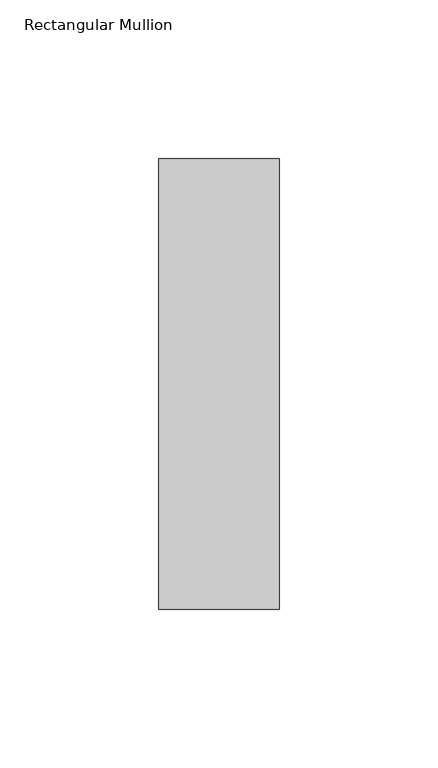
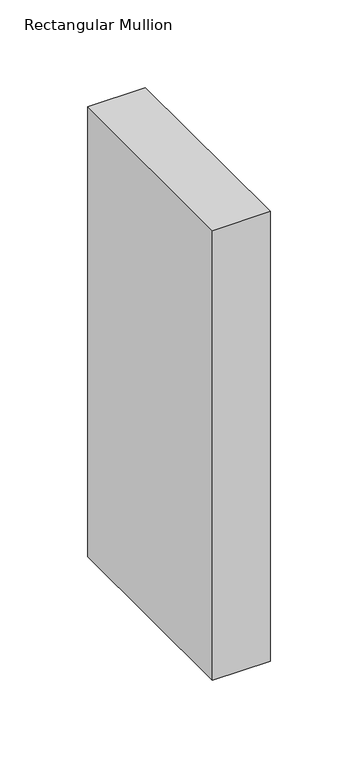
"""IFC4 building model written with IfcOpenShell, lengths in millimetres: member geometry, Rectangular Mullion : NLRS_21_CWM_hsb-regel 38x142_gen_rsf."""

from ifc_helpers import new_model, si_unit, frame, origin, place, context, project, spatial, polyline, outline, extrude, source, transform, mapped, element, save


def rectangular_mullion_533ed1c3(model_context):
    return source(origin(), model_context, "Body", "SweptSolid", [
        extrude(outline(polyline([(-38.0, -71.0), (-38.0, 71.0), (0.0, 71.0), (0.0, -71.0), (-38.0, -71.0)])), frame((0.0, 0.0, -312.8441061), z_axis=(0.0, 0.0, 1.0), x_axis=(1.0, 0.0, 0.0)), (0.0, 0.0, 1.0), 312.8441061),
    ])


if __name__ == "__main__":
    model = new_model("IFC4")
    model_context = context("Model", 3, world=origin())
    ifc_project = project(units=[si_unit("LENGTHUNIT", "METRE", prefix="MILLI")], contexts=[model_context])
    site = spatial("IfcSite", under=ifc_project)
    building = spatial("IfcBuilding", under=site)
    placement = place(None, origin())
    rectangular_mullion_shape = rectangular_mullion_533ed1c3(model_context)
    element("IfcMember", 1, ObjectType="Rectangular Mullion : NLRS_21_CWM_hsb-regel 38x142_gen_rsf", at=placement, inside=building, context=model_context, shape_type="MappedRepresentation", body=[
        mapped(rectangular_mullion_shape, transform((0.0, 0.0, 0.0), x_axis=(1.0, 0.0, 0.0), y_axis=(0.0, 1.0, 0.0), z_axis=(0.0, 0.0, 1.0))),
    ])
    save(model, "model.ifc")

# Revit data of these elements
# Type "Rectangular Mullion : NLRS_21_CWM_hsb-regel 38x142_gen_rsf"
#   Export Type to IFC As = "IfcWall"
#   Type IfcGUID = "07M7mRoiH1CR8m_RSKIwpF"
#   Assembly Code = "21.10"
#   built-in parameter 1007322 = 0.465879 (stored number, unit not read)
#   built-in parameter 1007321 = 0.062336 (stored number, unit not read)
#   built-in parameter 1007320 = 0.062336 (stored number, unit not read)
# Element 1 (IfcMember, "Rectangular Mullion : NLRS_21_CWM_hsb-regel 38x142_gen_rsf")
#   Materials on its faces: "NLRS_i2_hout naaldhout vuren_gen_rsf"
# Materials
#   "NLRS_i2_hout naaldhout vuren_gen_rsf": class "I - Hout", colour RGB 234 199 147, transparency 0, Keynote = "i2", Manufacturer = "Revit Standards Foundation", URL = "www.revitstandards.org", Description = "hout vuren", Cost = 0
